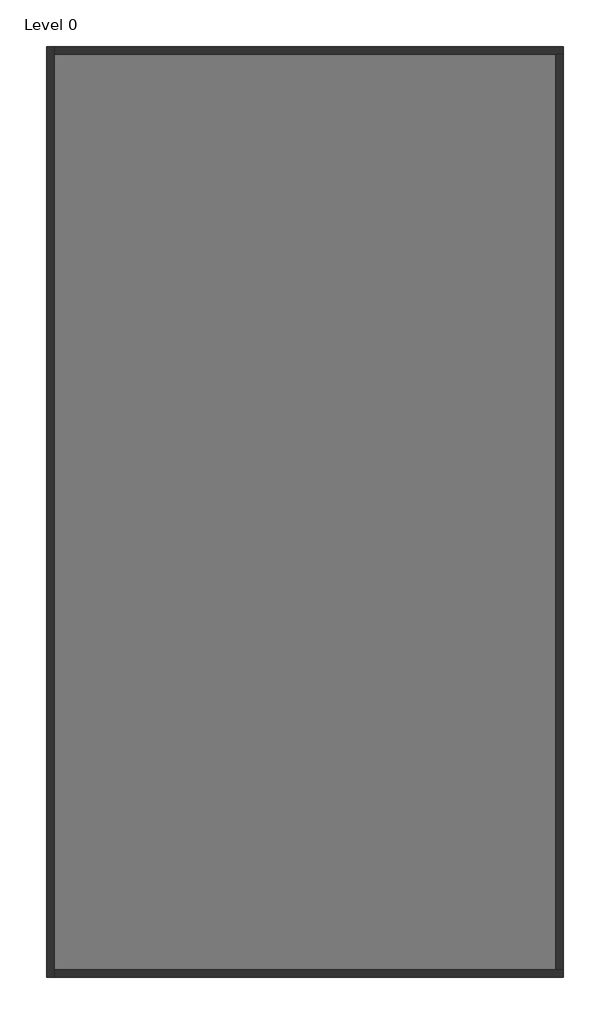
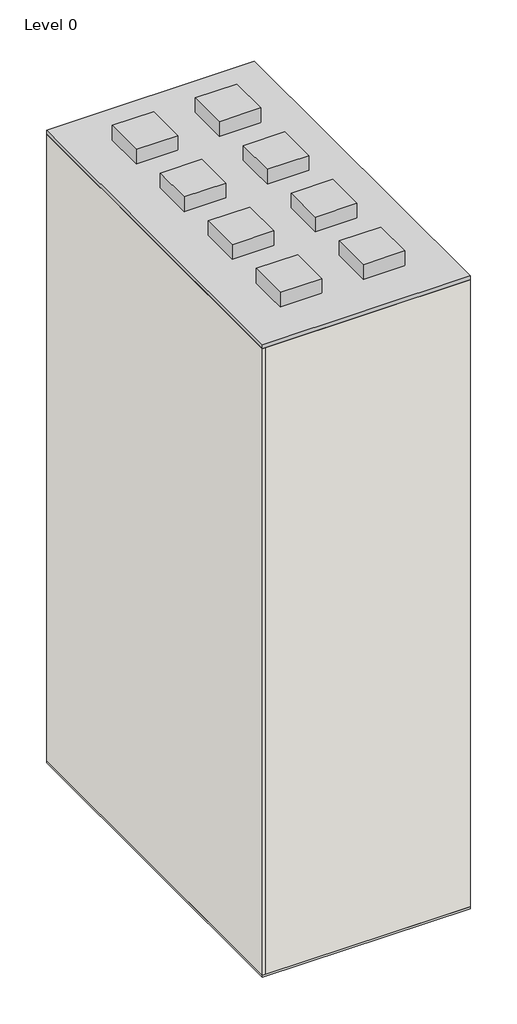
# One storey: 4 walls, 1 proxy, 1 slab.
"""IFC4 building model written with IfcOpenShell, lengths in millimetres."""

import ifcopenshell
import ifcopenshell.guid

model = None  # the IFC model being written
_history = None  # IfcOwnerHistory: only IFC2X3 demands one
_inside = {}  # id of a spatial element -> (the spatial element, [elements in it])
_under = {}  # id of a project, library or spatial element -> (it, [spatial elements below it])
_declared = {}  # id of a project -> (the project, [libraries it declares])
_typed = {}  # id of a type object -> (the type object, [elements of that type])
_made_of = {}  # id of a material, layer set ... -> (it, [elements and type objects made of it])


def new_model(schema):
    """Start an empty IFC model of exactly this schema.

    Asked for "IFC4X3", IfcOpenShell would pick the latest addendum, in which some entities
    have other attributes; the version numbers below select the first issue.
    IFC2X3 requires an IfcOwnerHistory on every rooted entity: one is made here for all.
    """
    global model, _history
    if schema == "IFC4X3":
        model = ifcopenshell.file(schema_version=(4, 3, 0, 0))
    else:
        model = ifcopenshell.file(schema=schema)
    _inside.clear()
    _under.clear()
    _declared.clear()
    _typed.clear()
    _made_of.clear()
    _history = None
    if model.schema == "IFC2X3":
        org = make("IfcOrganization", Name="unknown")
        user = make(
            "IfcPersonAndOrganization",
            ThePerson=make("IfcPerson", FamilyName="unknown"),
            TheOrganization=org,
        )
        app = make(
            "IfcApplication",
            ApplicationDeveloper=org,
            Version="unknown",
            ApplicationFullName="unknown",
            ApplicationIdentifier="unknown",
        )
        _history = make(
            "IfcOwnerHistory",
            OwningUser=user,
            OwningApplication=app,
            ChangeAction="ADDED",
            CreationDate=0,
        )
    return model


def make(cls, **values):
    """One entity of the class cls with the attributes given. An attribute that is None is left unset."""
    return model.create_entity(
        cls, **{name: value for name, value in values.items() if value is not None}
    )


def rooted(cls, **values):
    """An entity with a GlobalId (a new one), such as an element, a storey or a relation."""
    return make(cls, GlobalId=ifcopenshell.guid.new(), OwnerHistory=_history, **values)


def si_unit(unit_type, name, prefix=None):
    """IfcSIUnit, for example si_unit("LENGTHUNIT", "METRE", prefix="MILLI")."""
    return make("IfcSIUnit", UnitType=unit_type, Prefix=prefix, Name=name)


def assignment(units):
    """IfcUnitAssignment: the units of a project."""
    return None if units is None else make("IfcUnitAssignment", Units=units)


def point(xyz):
    """IfcCartesianPoint."""
    return None if xyz is None else make("IfcCartesianPoint", Coordinates=xyz)


def direction(xyz):
    """IfcDirection."""
    return None if xyz is None else make("IfcDirection", DirectionRatios=xyz)


def frame(location, z_axis=None, x_axis=None):
    """IfcAxis2Placement3D, a coordinate frame: its origin and axes. An axis left out is left unset."""
    return make(
        "IfcAxis2Placement3D",
        Location=point(location),
        Axis=direction(z_axis),
        RefDirection=direction(x_axis),
    )


def origin():
    """The frame at (0, 0, 0) with its axes left unset."""
    return frame((0.0, 0.0, 0.0))


def origin_with_axes():
    """The frame at (0, 0, 0) with the z axis (0, 0, 1) and the x axis (1, 0, 0) written out."""
    return frame((0.0, 0.0, 0.0), z_axis=(0.0, 0.0, 1.0), x_axis=(1.0, 0.0, 0.0))


def place(relative_to, where):
    """IfcLocalPlacement: puts the frame where relative to a parent placement (None: the world)."""
    return make(
        "IfcLocalPlacement", PlacementRelTo=relative_to, RelativePlacement=where
    )


def context(
    kind, dimensions, precision=None, world=None, true_north=None, identifier=None
):
    """IfcGeometricRepresentationContext, for example the 3D "Model" context."""
    return make(
        "IfcGeometricRepresentationContext",
        ContextIdentifier=identifier,
        ContextType=kind,
        CoordinateSpaceDimension=dimensions,
        Precision=precision,
        WorldCoordinateSystem=world,
        TrueNorth=true_north,
    )


def project(units=None, contexts=None):
    """IfcProject with its units and contexts."""
    return rooted(
        "IfcProject",
        Name="project",
        RepresentationContexts=contexts,
        UnitsInContext=assignment(units),
    )


def spatial(cls, under=None, at=None, **own):
    """A site, building, storey or space (cls), placed at a placement, below another one or the project."""
    s = rooted(cls, ObjectPlacement=at, **own)
    if under is not None:
        _under.setdefault(under.id(), (under, []))[1].append(s)
    return s


def polyline(points):
    """IfcPolyline through the points."""
    return make("IfcPolyline", Points=[point(p) for p in points])


def outline(outer, holes=None, kind="AREA"):
    """IfcArbitraryClosedProfileDef: a profile drawn as a closed curve; with holes, ...WithVoids."""
    if holes is None:
        return make("IfcArbitraryClosedProfileDef", ProfileType=kind, OuterCurve=outer)
    return make(
        "IfcArbitraryProfileDefWithVoids",
        ProfileType=kind,
        OuterCurve=outer,
        InnerCurves=holes,
    )


def extrude(swept, where, along, depth):
    """IfcExtrudedAreaSolid: the profile swept, set in the frame where, extruded along a direction by depth."""
    return make(
        "IfcExtrudedAreaSolid",
        SweptArea=swept,
        Position=where,
        ExtrudedDirection=direction(along),
        Depth=depth,
    )


def faces_of(points, faces, orient=None, outer=None):
    """IfcFace entities. A face is a list of loops; a loop is a list of indices into points, from 0.

    orient and outer hold one flag for each loop. By default every Orientation is true, the
    first loop of a face is its IfcFaceOuterBound and the others are IfcFaceBound.
    """
    made = []
    for i, loops in enumerate(faces):
        bounds = []
        for j, loop in enumerate(loops):
            is_outer = j == 0 if outer is None else outer[i][j]
            bounds.append(
                make(
                    "IfcFaceOuterBound" if is_outer else "IfcFaceBound",
                    Bound=make("IfcPolyLoop", Polygon=[points[k] for k in loop]),
                    Orientation=True if orient is None else orient[i][j],
                )
            )
        made.append(make("IfcFace", Bounds=bounds))
    return made


def faceted_brep(points, faces, orient=None, outer=None, voids=None):
    """IfcFacetedBrep: a solid bounded by flat faces; with voids (closed shells), ...WithVoids."""
    shared = [point(p) for p in points]
    hull = make("IfcClosedShell", CfsFaces=faces_of(shared, faces, orient, outer))
    if voids is None:
        return make("IfcFacetedBrep", Outer=hull)
    return make(
        "IfcFacetedBrepWithVoids",
        Outer=hull,
        Voids=[
            make(cls, CfsFaces=faces_of(shared, fs, o, b)) for cls, fs, o, b in voids
        ],
    )


def shape(context_of_items, identifier, shape_type, items):
    """IfcShapeRepresentation: the items that make up one representation, for example the "Body"."""
    return make(
        "IfcShapeRepresentation",
        ContextOfItems=context_of_items,
        RepresentationIdentifier=identifier,
        RepresentationType=shape_type,
        Items=items,
    )


def made_of(thing, what):
    """Note that an element or type object is made of a material, layer set ...; save() writes the relation."""
    if what is not None:
        _made_of.setdefault(what.id(), (what, []))[1].append(thing)
    return thing


def element(
    cls,
    number,
    at=None,
    inside=None,
    cuts=None,
    type_object=None,
    material=None,
    context=None,
    identifier="Body",
    shape_type=None,
    held_by="IfcProductDefinitionShape",
    body=None,
    shapes=None,
    **own,
):
    """One element of the class cls, such as IfcWall. Its Tag is "e" and its number.

    at: its placement. inside: the storey or other place that contains it. cuts: it is an
    opening in that element (IfcRelVoidsElement). A single representation is given by context,
    identifier, shape_type and body (its items); several are given by shapes. held_by: the class
    of the entity that holds the representations. save() writes the other relations.
    """
    e = rooted(cls, Tag="e%d" % number, ObjectPlacement=at, **own)
    if body is not None:
        shapes = [shape(context, identifier, shape_type, body)]
    if shapes is not None:
        e.Representation = make(held_by, Representations=shapes)
    if inside is not None:
        _inside.setdefault(inside.id(), (inside, []))[1].append(e)
    if cuts is not None:
        rooted(
            "IfcRelVoidsElement", RelatingBuildingElement=cuts, RelatedOpeningElement=e
        )
    if type_object is not None:
        _typed.setdefault(type_object.id(), (type_object, []))[1].append(e)
    return made_of(e, material)


def aggregate(whole, parts):
    """IfcRelAggregates: a whole, such as a stair, and the parts it consists of."""
    return rooted("IfcRelAggregates", RelatingObject=whole, RelatedObjects=parts)


def save(model, path):
    """Write the relations noted so far, then the file.

    IfcRelAggregates (storeys below a building ...), IfcRelContainedInSpatialStructure (elements
    in a storey), IfcRelDefinesByType, IfcRelAssociatesMaterial and IfcRelDeclares: one each for
    every whole, place, type object, material and project.
    """
    for whole, parts in _under.values():
        aggregate(whole, parts)
    for where, things in _inside.values():
        rooted(
            "IfcRelContainedInSpatialStructure",
            RelatedElements=things,
            RelatingStructure=where,
        )
    for kind, things in _typed.values():
        rooted("IfcRelDefinesByType", RelatedObjects=things, RelatingType=kind)
    for what, things in _made_of.values():
        rooted("IfcRelAssociatesMaterial", RelatedObjects=things, RelatingMaterial=what)
    for by, libraries in _declared.values():
        rooted("IfcRelDeclares", RelatingContext=by, RelatedDefinitions=libraries)
    model.write(path)


model = new_model("IFC4")

# Units and contexts
model_context = context("Model", 3, world=origin())
ifc_project = project(units=[si_unit("LENGTHUNIT", "METRE", prefix="MILLI")], contexts=[model_context])

# Site, building, storey
site = spatial("IfcSite", under=ifc_project)
building = spatial("IfcBuilding", under=site)
storey = spatial("IfcBuildingStorey", under=building, Name="Level 0", Elevation=100.0)

# Proxy
placement = place(None, origin())
element("IfcBuildingElementProxy", 1, Name="LowUrbanDensityBuilding : LowUrbanDensityBuilding", ObjectType="LowUrbanDensityBuilding : LowUrbanDensityBuilding", at=placement, inside=storey, context=model_context, shape_type="SweptSolid", body=[
    extrude(outline(polyline([(7325.2659446, 3676.2074539), (7325.2659446, -14323.7925461), (-2674.7340554, -14323.7925461), (-2674.7340554, 3676.2074539), (7325.2659446, 3676.2074539)])), origin_with_axes(), (0.0, 0.0, 1.0), 32200.0),
    extrude(outline(polyline([(1325.2659446, 1676.2074539), (1325.2659446, -323.7925461), (-674.7340554, -323.7925461), (-674.7340554, 1676.2074539), (1325.2659446, 1676.2074539)])), frame((0.0, 0.0, 32000.0), z_axis=(0.0, 0.0, 1.0), x_axis=(1.0, 0.0, 0.0)), (0.0, 0.0, 1.0), 949.8),
    extrude(outline(polyline([(5325.2659446, 1676.2074539), (5325.2659446, -323.7925461), (3325.2659446, -323.7925461), (3325.2659446, 1676.2074539), (5325.2659446, 1676.2074539)])), frame((0.0, 0.0, 32000.0), z_axis=(0.0, 0.0, 1.0), x_axis=(1.0, 0.0, 0.0)), (0.0, 0.0, 1.0), 949.8),
    extrude(outline(polyline([(1325.2659446, -2323.7925461), (1325.2659446, -4323.7925461), (-674.7340554, -4323.7925461), (-674.7340554, -2323.7925461), (1325.2659446, -2323.7925461)])), frame((0.0, 0.0, 32000.0), z_axis=(0.0, 0.0, 1.0), x_axis=(1.0, 0.0, 0.0)), (0.0, 0.0, 1.0), 949.8),
    extrude(outline(polyline([(5325.2659446, -2323.7925461), (5325.2659446, -4323.7925461), (3325.2659446, -4323.7925461), (3325.2659446, -2323.7925461), (5325.2659446, -2323.7925461)])), frame((0.0, 0.0, 32000.0), z_axis=(0.0, 0.0, 1.0), x_axis=(1.0, 0.0, 0.0)), (0.0, 0.0, 1.0), 949.8),
    extrude(outline(polyline([(1325.2659446, -6323.7925461), (1325.2659446, -8323.7925461), (-674.7340554, -8323.7925461), (-674.7340554, -6323.7925461), (1325.2659446, -6323.7925461)])), frame((0.0, 0.0, 32000.0), z_axis=(0.0, 0.0, 1.0), x_axis=(1.0, 0.0, 0.0)), (0.0, 0.0, 1.0), 949.8),
    extrude(outline(polyline([(5325.2659446, -6323.7925461), (5325.2659446, -8323.7925461), (3325.2659446, -8323.7925461), (3325.2659446, -6323.7925461), (5325.2659446, -6323.7925461)])), frame((0.0, 0.0, 32000.0), z_axis=(0.0, 0.0, 1.0), x_axis=(1.0, 0.0, 0.0)), (0.0, 0.0, 1.0), 949.8),
    extrude(outline(polyline([(1325.2659446, -10323.7925461), (1325.2659446, -12323.7925461), (-674.7340554, -12323.7925461), (-674.7340554, -10323.7925461), (1325.2659446, -10323.7925461)])), frame((0.0, 0.0, 32000.0), z_axis=(0.0, 0.0, 1.0), x_axis=(1.0, 0.0, 0.0)), (0.0, 0.0, 1.0), 949.8),
    extrude(outline(polyline([(5325.2659446, -10323.7925461), (5325.2659446, -12323.7925461), (3325.2659446, -12323.7925461), (3325.2659446, -10323.7925461), (5325.2659446, -10323.7925461)])), frame((0.0, 0.0, 32000.0), z_axis=(0.0, 0.0, 1.0), x_axis=(1.0, 0.0, 0.0)), (0.0, 0.0, 1.0), 949.8),
])

# Slab
element("IfcSlab", 2, ObjectType="Floor-Concrete_100Con", at=placement, inside=storey, context=model_context, shape_type="SweptSolid", body=[
    extrude(outline(polyline([(7325.2659446, 3676.2074539), (7325.2659446, -14323.7925461), (-2674.7340554, -14323.7925461), (-2674.7340554, 3676.2074539), (7325.2659446, 3676.2074539)])), origin_with_axes(), (0.0, 0.0, 1.0), 100.0),
])

# Walls
element("IfcWall", 3, ObjectType="Wall-Ext_25Rdr-100Blk-19P", at=placement, inside=storey, context=model_context, shape_type="Brep", body=[
    faceted_brep([(-2674.7340554, 3676.2074539, 100.0), (-2674.7340554, -14323.7925461, 100.0), (-2674.7340554, -14323.7925461, 32000.0), (-2674.7340554, 3676.2074539, 32000.0), (-2530.4340554, 3676.2074539, 100.0), (-2530.4340554, 3676.2074539, 32000.0), (-2530.4340554, 3531.9074539, 32000.0), (-2530.4340554, -14179.4925461, 32000.0), (-2530.4340554, -14323.7925461, 32000.0), (-2530.4340554, -14323.7925461, 100.0), (-2530.4340554, -14179.4925461, 100.0), (-2530.4340554, 3531.9074539, 100.0)], [[[0, 1, 2, 3]], [[4, 5, 6, 7, 8, 9, 10, 11]], [[1, 0, 4, 11, 10, 9]], [[3, 2, 8, 7, 6, 5]], [[2, 1, 9, 8]], [[0, 3, 5, 4]]]),
])
element("IfcWall", 4, ObjectType="Wall-Ext_25Rdr-100Blk-19P", at=placement, inside=storey, context=model_context, shape_type="Brep", body=[
    faceted_brep([(-2530.4340554, -14323.7925461, 100.0), (7325.2659446, -14323.7925461, 100.0), (7325.2659446, -14323.7925461, 32000.0), (-2530.4340554, -14323.7925461, 32000.0), (-2530.4340554, -14179.4925461, 100.0), (-2530.4340554, -14179.4925461, 32000.0), (7180.9659446, -14179.4925461, 32000.0), (7325.2659446, -14179.4925461, 32000.0), (7325.2659446, -14179.4925461, 100.0), (7180.9659446, -14179.4925461, 100.0)], [[[0, 1, 2, 3]], [[4, 5, 6, 7, 8, 9]], [[1, 0, 4, 9, 8]], [[3, 2, 7, 6, 5]], [[0, 3, 5, 4]], [[2, 1, 8, 7]]]),
])
element("IfcWall", 5, ObjectType="Wall-Ext_25Rdr-100Blk-19P", at=placement, inside=storey, context=model_context, shape_type="Brep", body=[
    faceted_brep([(7325.2659446, 3676.2074539, 100.0), (-2530.4340554, 3676.2074539, 100.0), (-2530.4340554, 3676.2074539, 32000.0), (7325.2659446, 3676.2074539, 32000.0), (7325.2659446, 3531.9074539, 100.0), (7325.2659446, 3531.9074539, 32000.0), (7180.9659446, 3531.9074539, 32000.0), (-2530.4340554, 3531.9074539, 32000.0), (-2530.4340554, 3531.9074539, 100.0), (7180.9659446, 3531.9074539, 100.0)], [[[0, 1, 2, 3]], [[4, 5, 6, 7, 8, 9]], [[1, 0, 4, 9, 8]], [[3, 2, 7, 6, 5]], [[2, 1, 8, 7]], [[0, 3, 5, 4]]]),
])
element("IfcWall", 6, ObjectType="Wall-Ext_25Rdr-100Blk-19P", at=placement, inside=storey, context=model_context, shape_type="SweptSolid", body=[
    extrude(outline(polyline([(7325.2659446, 3531.9074539), (7325.2659446, -14179.4925461), (7180.9659446, -14179.4925461), (7180.9659446, 3531.9074539), (7325.2659446, 3531.9074539)])), frame((0.0, 0.0, 100.0), z_axis=(0.0, 0.0, 1.0), x_axis=(1.0, 0.0, 0.0)), (0.0, 0.0, 1.0), 31900.0),
])

save(model, "model.ifc")

# Revit data of these elements
# Project information
#   Project Issue Date = "Issue Date"
#   Project Status = "Project Status"
#   Client Name = "Owner"
#   Project Address = "Enter address here"
#   Project Name = "Project Name"
#   Project Number = "Project Number"
# Type "Floor-Concrete_100Con"
#   Keynote = "E60/130"
#   Function = 0
#   Layers, outside or top first: 100 mm "Concrete" (function 1)
# Type "Wall-Ext_25Rdr-100Blk-19P"
#   Keynote = "F10"
#   Layers, outside or top first: 25.3 mm "Render, Beige, Smooth" (function 5); 100 mm "Concrete Masonry Units _Low Density" (function 1); 19 mm "Plaster" (function 5)
# Element 1 (IfcBuildingElementProxy, "LowUrbanDensityBuilding : LowUrbanDensityBuilding")
#   Phase Created = New Construction
#   Materials on its faces: "Default Form"
# Element 2 (IfcSlab, "Floor-Concrete_100Con")
#   Height Offset From Level = 0 mm
#   Phase Created = New Construction
#   Materials on its faces: "Concrete"
# Element 3 (IfcWall, "Wall-Ext_25Rdr-100Blk-19P")
#   Top Offset = 0 mm
#   Base Offset = 0 mm
#   wall height = 31900 mm
#   Phase Created = New Construction
#   Base Constraint = Level 0
#   Top Constraint = Level 8
#   Materials on its faces: "Render, Beige, Smooth", "Default Wall", "Plaster"
# Elements 4, 5, 6 (IfcWall, "Wall-Ext_25Rdr-100Blk-19P")
#   Top Offset = 0 mm
#   Base Offset = 0 mm
#   wall height = 31900 mm
#   Phase Created = New Construction
#   Base Constraint = Level 0
#   Top Constraint = Level 8
#   Materials on its faces: "Default Wall", "Render, Beige, Smooth", "Plaster"
# Materials
#   "Concrete": class "Concrete", colour RGB 120 120 120, transparency 0, Description = "Portland Cement Concrete", Cost = 0
#   "Render, Beige, Smooth": class "Generic", colour RGB 213 198 180, transparency 0, Description = "physical material", Cost = 0
#   "Concrete Masonry Units _Low Density": class "Masonry", colour RGB 181 181 181, transparency 0, Description = "Concrete masonry units", Cost = 0
#   "Plaster": class "Generic", colour RGB 249 249 249, transparency 0, Description = "Plaster", Cost = 0
#   "Default Form": class "Generic", colour RGB 185 189 196, transparency 0.5, Cost = 0
#   "Default Wall": class "Miscellaneous", colour RGB 128 128 128, transparency 0, Comments = "Rendering appearance not upgraded Rendering appearance not upgraded ", Cost = 0
